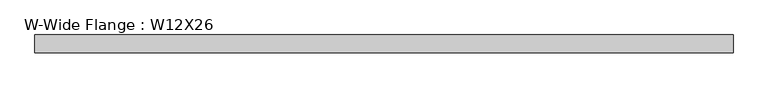
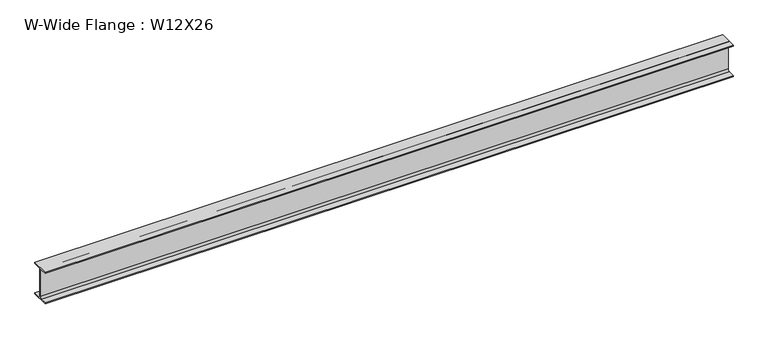
"""IFC4 building model written with IfcOpenShell, lengths in millimetres: beam geometry, W-Wide Flange : W12X26."""

from ifc_helpers import new_model, si_unit, point, frame, frame_2d, origin, place, context, project, spatial, polyline, circle_curve, trimmed, segment, composite_curve, outline, extrude, source, transform, mapped, element, save


def w_wide_flange_w12x26_3769b023(model_context):
    return source(origin(), model_context, "Body", "SweptSolid", [
        extrude(outline(composite_curve([segment(polyline([(82.4011719, -145.5539063), (82.4011719, -155.178125), (-82.4011719, -155.178125), (-82.4011719, -145.5539063), (-20.2902344, -145.5539063)]), True, "CONTINUOUS"), segment(trimmed(circle_curve(frame_2d((-20.2902344, -128.190625)), 17.3632812), [point((-20.2902344, -145.5539063))], [point((-2.9269531, -128.190625))], True, "CARTESIAN"), True, "CONTINUOUS"), segment(polyline([(-2.9269531, -128.190625), (-2.9269531, 128.190625)]), True, "CONTINUOUS"), segment(trimmed(circle_curve(frame_2d((-20.2902344, 128.190625)), 17.3632812), [point((-2.9269531, 128.190625))], [point((-20.2902344, 145.5539062))], True, "CARTESIAN"), True, "CONTINUOUS"), segment(polyline([(-20.2902344, 145.5539062), (-82.4011719, 145.5539062), (-82.4011719, 155.178125), (82.4011719, 155.178125), (82.4011719, 145.5539062), (20.2902344, 145.5539062)]), True, "CONTINUOUS"), segment(trimmed(circle_curve(frame_2d((20.2902344, 128.190625)), 17.3632812), [point((20.2902344, 145.5539062))], [point((2.9269531, 128.190625))], True, "CARTESIAN"), True, "CONTINUOUS"), segment(polyline([(2.9269531, 128.190625), (2.9269531, -128.190625)]), True, "CONTINUOUS"), segment(trimmed(circle_curve(frame_2d((20.2902344, -128.190625)), 17.3632812), [point((2.9269531, -128.190625))], [point((20.2902344, -145.5539063))], True, "CARTESIAN"), True, "CONTINUOUS"), segment(polyline([(20.2902344, -145.5539063), (82.4011719, -145.5539063)]), True, "CONTINUOUS")], self_intersect=False)), frame((-3333.7106844, 0.0, 0.0), z_axis=(1.0, 0.0, 0.0), x_axis=(0.0, 1.0, 0.0)), (0.0, 0.0, 1.0), 6397.5856844),
    ])


if __name__ == "__main__":
    model = new_model("IFC4")
    model_context = context("Model", 3, world=origin())
    ifc_project = project(units=[si_unit("LENGTHUNIT", "METRE", prefix="MILLI")], contexts=[model_context])
    site = spatial("IfcSite", under=ifc_project)
    building = spatial("IfcBuilding", under=site)
    placement = place(None, origin())
    w_wide_flange_w12x26_shape = w_wide_flange_w12x26_3769b023(model_context)
    element("IfcBeam", 1, ObjectType="W-Wide Flange : W12X26", at=placement, inside=building, context=model_context, shape_type="MappedRepresentation", body=[
        mapped(w_wide_flange_w12x26_shape, transform((0.0, 0.0, 0.0), x_axis=(1.0, 0.0, 0.0), y_axis=(0.0, 1.0, 0.0), z_axis=(0.0, 0.0, 1.0))),
    ])
    save(model, "model.ifc")

# Revit data of these elements
# Type "W-Wide Flange : W12X26"
#   Assembly Code = "B10"
#   W = 26
#   Length [instance default] = 5' - 0"
#   bf = 0' - 6 125/256"
#   d = 1' - 0 7/32"
#   k = 0' - 1 1/16"
#   k2 = 0' - 0 175/256"
#   tf = 0' - 0 97/256"
#   tw = 0' - 0 59/256"
#   A = 0.053125 SF
#   Structural Material [instance default] = Steel ASTM A992
# Element 1 (IfcBeam, "W-Wide Flange : W12X26")
#   Structural Material = STRUCTURAL STEEL - SEE STRUCT. DWGS
#   Materials on its faces: "STRUCTURAL STEEL - SEE STRUCT. DWGS"
# Materials
#   "Steel ASTM A992": class "Metal", colour RGB 199 199 199, transparency 0, Description = "Structural steel 50ksi", Cost = 0
#   "STRUCTURAL STEEL - SEE STRUCT. DWGS": class "Metal", colour RGB 137 146 153, transparency 0, Description = "Steel, mill finish", Cost = 0
